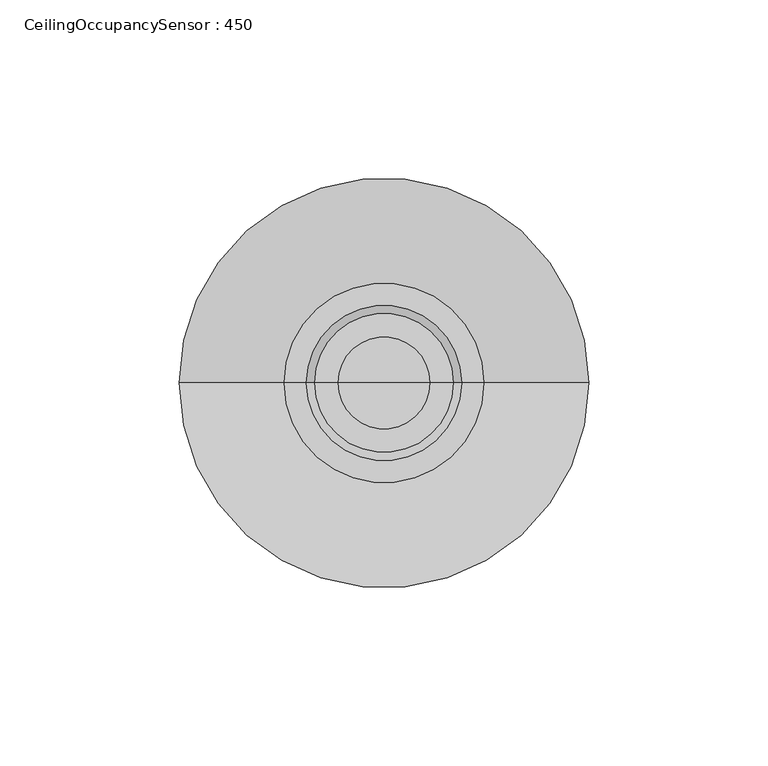
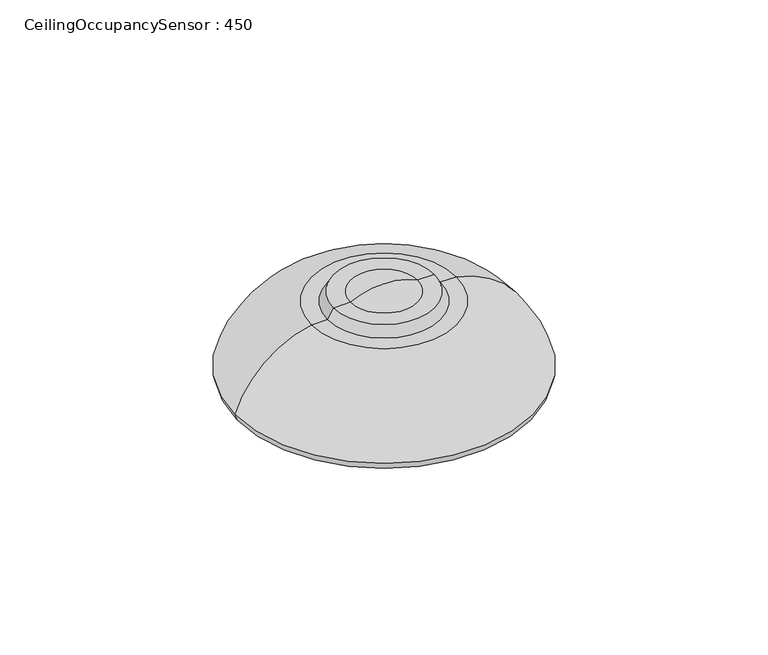
"""IFC4 building model written with IfcOpenShell, lengths in millimetres: switching device geometry, CeilingOccupancySensor : 450."""

import ifcopenshell
import ifcopenshell.guid

model = None  # the IFC model being written
_history = None  # IfcOwnerHistory: only IFC2X3 demands one
_inside = {}  # id of a spatial element -> (the spatial element, [elements in it])
_under = {}  # id of a project, library or spatial element -> (it, [spatial elements below it])
_declared = {}  # id of a project -> (the project, [libraries it declares])
_typed = {}  # id of a type object -> (the type object, [elements of that type])
_made_of = {}  # id of a material, layer set ... -> (it, [elements and type objects made of it])


def new_model(schema):
    """Start an empty IFC model of exactly this schema.

    Asked for "IFC4X3", IfcOpenShell would pick the latest addendum, in which some entities
    have other attributes; the version numbers below select the first issue.
    IFC2X3 requires an IfcOwnerHistory on every rooted entity: one is made here for all.
    """
    global model, _history
    if schema == "IFC4X3":
        model = ifcopenshell.file(schema_version=(4, 3, 0, 0))
    else:
        model = ifcopenshell.file(schema=schema)
    _inside.clear()
    _under.clear()
    _declared.clear()
    _typed.clear()
    _made_of.clear()
    _history = None
    if model.schema == "IFC2X3":
        org = make("IfcOrganization", Name="unknown")
        user = make(
            "IfcPersonAndOrganization",
            ThePerson=make("IfcPerson", FamilyName="unknown"),
            TheOrganization=org,
        )
        app = make(
            "IfcApplication",
            ApplicationDeveloper=org,
            Version="unknown",
            ApplicationFullName="unknown",
            ApplicationIdentifier="unknown",
        )
        _history = make(
            "IfcOwnerHistory",
            OwningUser=user,
            OwningApplication=app,
            ChangeAction="ADDED",
            CreationDate=0,
        )
    return model


def make(cls, **values):
    """One entity of the class cls with the attributes given. An attribute that is None is left unset."""
    return model.create_entity(
        cls, **{name: value for name, value in values.items() if value is not None}
    )


def rooted(cls, **values):
    """An entity with a GlobalId (a new one), such as an element, a storey or a relation."""
    return make(cls, GlobalId=ifcopenshell.guid.new(), OwnerHistory=_history, **values)


def si_unit(unit_type, name, prefix=None):
    """IfcSIUnit, for example si_unit("LENGTHUNIT", "METRE", prefix="MILLI")."""
    return make("IfcSIUnit", UnitType=unit_type, Prefix=prefix, Name=name)


def assignment(units):
    """IfcUnitAssignment: the units of a project."""
    return None if units is None else make("IfcUnitAssignment", Units=units)


def point(xyz):
    """IfcCartesianPoint."""
    return None if xyz is None else make("IfcCartesianPoint", Coordinates=xyz)


def direction(xyz):
    """IfcDirection."""
    return None if xyz is None else make("IfcDirection", DirectionRatios=xyz)


def frame(location, z_axis=None, x_axis=None):
    """IfcAxis2Placement3D, a coordinate frame: its origin and axes. An axis left out is left unset."""
    return make(
        "IfcAxis2Placement3D",
        Location=point(location),
        Axis=direction(z_axis),
        RefDirection=direction(x_axis),
    )


def origin():
    """The frame at (0, 0, 0) with its axes left unset."""
    return frame((0.0, 0.0, 0.0))


def origin_with_axes():
    """The frame at (0, 0, 0) with the z axis (0, 0, 1) and the x axis (1, 0, 0) written out."""
    return frame((0.0, 0.0, 0.0), z_axis=(0.0, 0.0, 1.0), x_axis=(1.0, 0.0, 0.0))


def place(relative_to, where):
    """IfcLocalPlacement: puts the frame where relative to a parent placement (None: the world)."""
    return make(
        "IfcLocalPlacement", PlacementRelTo=relative_to, RelativePlacement=where
    )


def context(
    kind, dimensions, precision=None, world=None, true_north=None, identifier=None
):
    """IfcGeometricRepresentationContext, for example the 3D "Model" context."""
    return make(
        "IfcGeometricRepresentationContext",
        ContextIdentifier=identifier,
        ContextType=kind,
        CoordinateSpaceDimension=dimensions,
        Precision=precision,
        WorldCoordinateSystem=world,
        TrueNorth=true_north,
    )


def project(units=None, contexts=None):
    """IfcProject with its units and contexts."""
    return rooted(
        "IfcProject",
        Name="project",
        RepresentationContexts=contexts,
        UnitsInContext=assignment(units),
    )


def spatial(cls, under=None, at=None, **own):
    """A site, building, storey or space (cls), placed at a placement, below another one or the project."""
    s = rooted(cls, ObjectPlacement=at, **own)
    if under is not None:
        _under.setdefault(under.id(), (under, []))[1].append(s)
    return s


def polyline(points):
    """IfcPolyline through the points."""
    return make("IfcPolyline", Points=[point(p) for p in points])


def circle_curve(where, radius):
    """IfcCircle in the frame where."""
    return make("IfcCircle", Position=where, Radius=radius)


def ellipse_curve(where, semi_axis1, semi_axis2):
    """IfcEllipse in the frame where."""
    return make(
        "IfcEllipse", Position=where, SemiAxis1=semi_axis1, SemiAxis2=semi_axis2
    )


def trimmed(basis, trim1, trim2, sense, master):
    """IfcTrimmedCurve: the piece of a basis curve between two trims."""
    return make(
        "IfcTrimmedCurve",
        BasisCurve=basis,
        Trim1=trim1,
        Trim2=trim2,
        SenseAgreement=sense,
        MasterRepresentation=master,
    )


def shape(context_of_items, identifier, shape_type, items):
    """IfcShapeRepresentation: the items that make up one representation, for example the "Body"."""
    return make(
        "IfcShapeRepresentation",
        ContextOfItems=context_of_items,
        RepresentationIdentifier=identifier,
        RepresentationType=shape_type,
        Items=items,
    )


def source(mapping_origin, context_of_items, identifier, shape_type, items):
    """IfcRepresentationMap: a shape defined once, which mapped items show again and again."""
    return make(
        "IfcRepresentationMap",
        MappingOrigin=mapping_origin,
        MappedRepresentation=shape(context_of_items, identifier, shape_type, items),
    )


def transform(
    local_origin,
    x_axis=None,
    y_axis=None,
    z_axis=None,
    scale=None,
    scale2=None,
    scale3=None,
    uniform=True,
):
    """IfcCartesianTransformationOperator3D, or its non-uniform kind. x_axis, y_axis, z_axis: its Axis1, 2, 3."""
    if uniform:
        return make(
            "IfcCartesianTransformationOperator3D",
            Axis1=direction(x_axis),
            Axis2=direction(y_axis),
            LocalOrigin=point(local_origin),
            Scale=scale,
            Axis3=direction(z_axis),
        )
    return make(
        "IfcCartesianTransformationOperator3DnonUniform",
        Axis1=direction(x_axis),
        Axis2=direction(y_axis),
        LocalOrigin=point(local_origin),
        Scale=scale,
        Axis3=direction(z_axis),
        Scale2=scale2,
        Scale3=scale3,
    )


def mapped(mapping_source, mapping_target):
    """IfcMappedItem: shows the shape of a source again, moved by a transform."""
    return make(
        "IfcMappedItem", MappingSource=mapping_source, MappingTarget=mapping_target
    )


def made_of(thing, what):
    """Note that an element or type object is made of a material, layer set ...; save() writes the relation."""
    if what is not None:
        _made_of.setdefault(what.id(), (what, []))[1].append(thing)
    return thing


def element(
    cls,
    number,
    at=None,
    inside=None,
    cuts=None,
    type_object=None,
    material=None,
    context=None,
    identifier="Body",
    shape_type=None,
    held_by="IfcProductDefinitionShape",
    body=None,
    shapes=None,
    **own,
):
    """One element of the class cls, such as IfcWall. Its Tag is "e" and its number.

    at: its placement. inside: the storey or other place that contains it. cuts: it is an
    opening in that element (IfcRelVoidsElement). A single representation is given by context,
    identifier, shape_type and body (its items); several are given by shapes. held_by: the class
    of the entity that holds the representations. save() writes the other relations.
    """
    e = rooted(cls, Tag="e%d" % number, ObjectPlacement=at, **own)
    if body is not None:
        shapes = [shape(context, identifier, shape_type, body)]
    if shapes is not None:
        e.Representation = make(held_by, Representations=shapes)
    if inside is not None:
        _inside.setdefault(inside.id(), (inside, []))[1].append(e)
    if cuts is not None:
        rooted(
            "IfcRelVoidsElement", RelatingBuildingElement=cuts, RelatedOpeningElement=e
        )
    if type_object is not None:
        _typed.setdefault(type_object.id(), (type_object, []))[1].append(e)
    return made_of(e, material)


def aggregate(whole, parts):
    """IfcRelAggregates: a whole, such as a stair, and the parts it consists of."""
    return rooted("IfcRelAggregates", RelatingObject=whole, RelatedObjects=parts)


def save(model, path):
    """Write the relations noted so far, then the file.

    IfcRelAggregates (storeys below a building ...), IfcRelContainedInSpatialStructure (elements
    in a storey), IfcRelDefinesByType, IfcRelAssociatesMaterial and IfcRelDeclares: one each for
    every whole, place, type object, material and project.
    """
    for whole, parts in _under.values():
        aggregate(whole, parts)
    for where, things in _inside.values():
        rooted(
            "IfcRelContainedInSpatialStructure",
            RelatedElements=things,
            RelatingStructure=where,
        )
    for kind, things in _typed.values():
        rooted("IfcRelDefinesByType", RelatedObjects=things, RelatingType=kind)
    for what, things in _made_of.values():
        rooted("IfcRelAssociatesMaterial", RelatedObjects=things, RelatingMaterial=what)
    for by, libraries in _declared.values():
        rooted("IfcRelDeclares", RelatingContext=by, RelatedDefinitions=libraries)
    model.write(path)


def plane_surface(at):
    """IfcPlane: the flat surface through the origin of the frame at, square to its z axis."""
    return make("IfcPlane", Position=at)


def revolved_surface(curve, axis_point, axis_direction):
    """IfcSurfaceOfRevolution: the curve turned about the line through axis_point along axis_direction."""
    return make(
        "IfcSurfaceOfRevolution",
        SweptCurve=make("IfcArbitraryOpenProfileDef", ProfileType="CURVE", Curve=curve),
        AxisPosition=make("IfcAxis1Placement", Location=point(axis_point), Axis=direction(axis_direction)),
    )


def advanced_brep(points, edges, surfaces, faces):
    """IfcAdvancedBrep: a solid bounded by faces that lie on surfaces and meet in shared edges.

    An edge is (start, end): straight between two places in points (the first is 0);
    or (start, end, curve); or (start, end, curve, False) where it runs against its curve.
    A face is (place in surfaces, loops), or (place, loops, False) where it looks against
    its surface's normal. A loop lists edges by number (the first is 1), with a minus sign
    where the edge is run from its end to its start. The first loop is the outer one.
    """
    corners = [point(p) for p in points]
    vertices = [make("IfcVertexPoint", VertexGeometry=c) for c in corners]
    made = []
    for start, end, *more in edges:
        made.append(
            make(
                "IfcEdgeCurve",
                EdgeStart=vertices[start],
                EdgeEnd=vertices[end],
                EdgeGeometry=more[0] if more else make("IfcPolyline", Points=[corners[start], corners[end]]),
                SameSense=more[1] if len(more) > 1 else True,
            )
        )
    hull = []
    for where, loops, *sense in faces:
        bounds = []
        for j, loop in enumerate(loops):
            ring = [make("IfcOrientedEdge", EdgeElement=made[abs(k) - 1], Orientation=k > 0) for k in loop]
            bounds.append(
                make(
                    "IfcFaceOuterBound" if j == 0 else "IfcFaceBound",
                    Bound=make("IfcEdgeLoop", EdgeList=ring),
                    Orientation=True,
                )
            )
        hull.append(make("IfcAdvancedFace", Bounds=bounds, FaceSurface=surfaces[where], SameSense=sense[0] if sense else True))
    return make("IfcAdvancedBrep", Outer=make("IfcClosedShell", CfsFaces=hull))


def ceilingoccupancysensor_450_02cbfb90(model_context):
    return source(origin(), model_context, "Body", "AdvancedBrep", [
        advanced_brep(
        [(-12.7998992, 0.0, 32.54375), (12.7998992, 0.0, 32.54375), (0.0, 0.0, 35.5203125), (-19.3725919, 0.0, 32.54375), (19.3725919, 0.0, 32.54375), (-21.6519708, 0.0, 28.5957499), (21.6519708, 0.0, 28.5957499), (-27.834758, 0.0, 28.5957499), (27.834758, 0.0, 28.5957499), (-57.15, 0.0, 2.3911967), (57.15, 0.0, 2.3911967), (-56.5092808, 0.0, 0.0), (56.5092808, 0.0, 0.0), (0.0, 0.0, 0.0)],
        [
            (0, 1, circle_curve(frame((0.0, 0.0, 32.54375), z_axis=(0.0, 0.0, 1.0), x_axis=(1.0, 0.0, 0.0)), 12.7998992)),
            (1, 2, circle_curve(frame((0.750087, 0.0, 9.7363307), z_axis=(0.0, -1.0, 0.0), x_axis=(1.0, 0.0, 0.0)), 25.79489)),
            (2, 0, circle_curve(frame((-0.750087, 0.0, 9.7363307), z_axis=(0.0, -1.0, 0.0), x_axis=(-1.0, 0.0, 0.0)), 25.79489)),
            (1, 0, circle_curve(frame((0.0, 0.0, 32.54375), z_axis=(0.0, 0.0, 1.0), x_axis=(1.0, 0.0, 0.0)), 12.7998992)),
            (3, 4, circle_curve(frame((0.0, 0.0, 32.54375), z_axis=(0.0, 0.0, 1.0), x_axis=(1.0, 0.0, 0.0)), 19.3725919)),
            (4, 1),
            (0, 3),
            (4, 3, circle_curve(frame((0.0, 0.0, 32.54375), z_axis=(0.0, 0.0, 1.0), x_axis=(1.0, 0.0, 0.0)), 19.3725919)),
            (5, 6, circle_curve(frame((0.0, 0.0, 28.5957499), z_axis=(0.0, 0.0, 1.0), x_axis=(1.0, 0.0, 0.0)), 21.6519708)),
            (6, 4),
            (3, 5),
            (6, 5, circle_curve(frame((0.0, 0.0, 28.5957499), z_axis=(0.0, 0.0, 1.0), x_axis=(1.0, 0.0, 0.0)), 21.6519708)),
            (7, 8, circle_curve(frame((0.0, 0.0, 28.5957499), z_axis=(0.0, 0.0, 1.0), x_axis=(1.0, 0.0, 0.0)), 27.834758)),
            (8, 6),
            (5, 7),
            (8, 7, circle_curve(frame((0.0, 0.0, 28.5957499), z_axis=(0.0, 0.0, 1.0), x_axis=(1.0, 0.0, 0.0)), 27.834758)),
            (9, 10, circle_curve(frame((0.0, 0.0, 2.3911967), z_axis=(0.0, 0.0, 1.0), x_axis=(1.0, 0.0, 0.0)), 57.15)),
            (10, 8, circle_curve(frame((20.1846327, 0.0, -9.4623798), z_axis=(0.0, -1.0, 0.0), x_axis=(1.0, 0.0, 0.0)), 38.8193979)),
            (7, 9, circle_curve(frame((-20.1846327, 0.0, -9.4623798), z_axis=(0.0, -1.0, 0.0), x_axis=(-1.0, 0.0, 0.0)), 38.8193979)),
            (10, 9, circle_curve(frame((0.0, 0.0, 2.3911967), z_axis=(0.0, 0.0, 1.0), x_axis=(1.0, 0.0, 0.0)), 57.15)),
            (11, 12, circle_curve(origin_with_axes(), 56.5092808)),
            (12, 10),
            (9, 11),
            (12, 11, circle_curve(origin_with_axes(), 56.5092808)),
            (13, 12),
            (11, 13),
        ],
        [
            revolved_surface(trimmed(ellipse_curve(frame((0.750087, 0.0, 9.7363307), z_axis=(0.0, 1.0, 0.0), x_axis=(1.0, 0.0, 0.0)), 25.79489, 25.79489), [point((0.0, 0.0, 35.5203125))], [point((12.7998992, 0.0, 32.54375))], True, "CARTESIAN"), (0.0, 0.0, 38.1), (0.0, 0.0, -1.0)),
            plane_surface(frame((0.0, 0.0, 32.54375), z_axis=(0.0, 0.0, 1.0), x_axis=(1.0, 0.0, 0.0))),
            revolved_surface(polyline([(19.3725919, 0.0, 32.54375), (21.6519708, 0.0, 28.5957499)]), (0.0, 0.0, 38.1), (0.0, 0.0, -1.0)),
            plane_surface(frame((0.0, 0.0, 28.5957499), z_axis=(0.0, 0.0, 1.0), x_axis=(1.0, 0.0, 0.0))),
            revolved_surface(trimmed(ellipse_curve(frame((20.1846327, 0.0, -9.4623798), z_axis=(0.0, 1.0, 0.0), x_axis=(1.0, 0.0, 0.0)), 38.8193979, 38.8193979), [point((27.834758, 0.0, 28.5957499))], [point((57.15, 0.0, 2.3911967))], True, "CARTESIAN"), (0.0, 0.0, 38.1), (0.0, 0.0, -1.0)),
            revolved_surface(polyline([(57.15, 0.0, 2.3911967), (56.5092808, 0.0, 0.0)]), (0.0, 0.0, 38.1), (0.0, 0.0, -1.0)),
            plane_surface(frame((0.0, 0.0, 0.0), z_axis=(0.0, 0.0, -1.0), x_axis=(1.0, 0.0, 0.0))),
        ],
        [
            (0, [[1, 2, 3]]),
            (0, [[4, -3, -2]]),
            (1, [[5, 6, -1, 7]]),
            (1, [[8, -7, -4, -6]]),
            (2, [[9, 10, -5, 11]]),
            (2, [[12, -11, -8, -10]]),
            (3, [[13, 14, -9, 15]]),
            (3, [[16, -15, -12, -14]]),
            (4, [[17, 18, -13, 19]]),
            (4, [[20, -19, -16, -18]]),
            (5, [[21, 22, -17, 23]]),
            (5, [[24, -23, -20, -22]]),
            (6, [[25, -21, 26]]),
            (6, [[-26, -24, -25]]),
        ],
    ),
    ])


if __name__ == "__main__":
    model = new_model("IFC4")
    model_context = context("Model", 3, world=origin())
    ifc_project = project(units=[si_unit("LENGTHUNIT", "METRE", prefix="MILLI")], contexts=[model_context])
    site = spatial("IfcSite", under=ifc_project)
    building = spatial("IfcBuilding", under=site)
    placement = place(None, origin())
    ceilingoccupancysensor_450_shape = ceilingoccupancysensor_450_02cbfb90(model_context)
    element("IfcSwitchingDevice", 1, ObjectType="CeilingOccupancySensor : 450", at=placement, inside=building, context=model_context, shape_type="MappedRepresentation", body=[
        mapped(ceilingoccupancysensor_450_shape, transform((0.0, 0.0, 0.0), x_axis=(1.0, 0.0, 0.0), y_axis=(0.0, 1.0, 0.0), z_axis=(0.0, 0.0, 1.0))),
    ])
    save(model, "model.ifc")

# Revit data of these elements
# Type "CeilingOccupancySensor : 450"
#   Type Mark = "CeilingOccupancySensor"
#   Classification.OmniClass.21.Number = "21-04 50 40 10"
#   Classification.OmniClass.21.Description = "Lighting Control"
#   Classification.UniFormat.II.Description = "Lighting Control"
#   Classification.OmniClass.23.Number = "23-29 11 23 17"
#   Classification.OmniClass.23.Description = "Intrusion Detection Photoelectric Sensors"
#   Classification.UniFormat.II.Number = "D5040.10"
#   COBie.Type.CreatedBy = "info@mma.ie"
#   COBie.Type.CreatedOn = "2017-07-25T10:15:16"
#   COBie.Type.Name = "CeilingOccupancySensor"
#   COBie.Type.Category = "23-29 11 23 17 : Intrusion Detection Photoelectric Sensors"
#   COBie.Type.Description = "CeilingOccupancySensor_450"
#   COBie.Type.AssetType = "Fixed"
#   COBie.Type.Manufacturer = ""
#   COBie.Type.ModelNumber = ""
#   Voltage Comments = "20-24VDC"
#   Series = ""
#   Product URL = ""
#   Keynote = "28 16 19.A"
#   Copyright = ""
#   CADworks URL = ""
#   C.O.S. Material = "Plastic-White-Gloss"
#   Assembly Code = "D5030800"
#   COBie.Type.ReplacementCost = 0
#   Switch Voltage = 230 V
#   Nominal Width = 114.3 mm
#   Nominal Length = 114.3 mm
#   Nominal Depth = 35.52 mm
#   Minor Motion Detection = 1981.2 mm
#   Major Motion Detection = 3657.6 mm
#   Field of View = 360.00°
#   Coverage = 41.8064 m²
#   C.O.S. Field of View = 360.00°
#   C.O.S. Coverage = 41.8064 m²
#   COBie.Type = yes
#   Light Source [instance default] = yes
#   Infrared Minor Motion [instance default] = no
#   Infrared Major Motion [instance default] = no
#   Ballast Number of Poles = 1
#   Sensor Material = Plastic-White-Gloss
#   URL = ""
#   Type Comments = ""
#   Model = ""
#   Manufacturer = ""
#   Description = (empty or 0)
#   Default Elevation = 0
# Element 1 (IfcSwitchingDevice, "CeilingOccupancySensor : 450")
#   Materials on its faces: "Plastic-White-Gloss"
# Materials
#   "Plastic-White-Gloss": class "Plastic", colour RGB 255 255 255, transparency 0, Cost = 0
